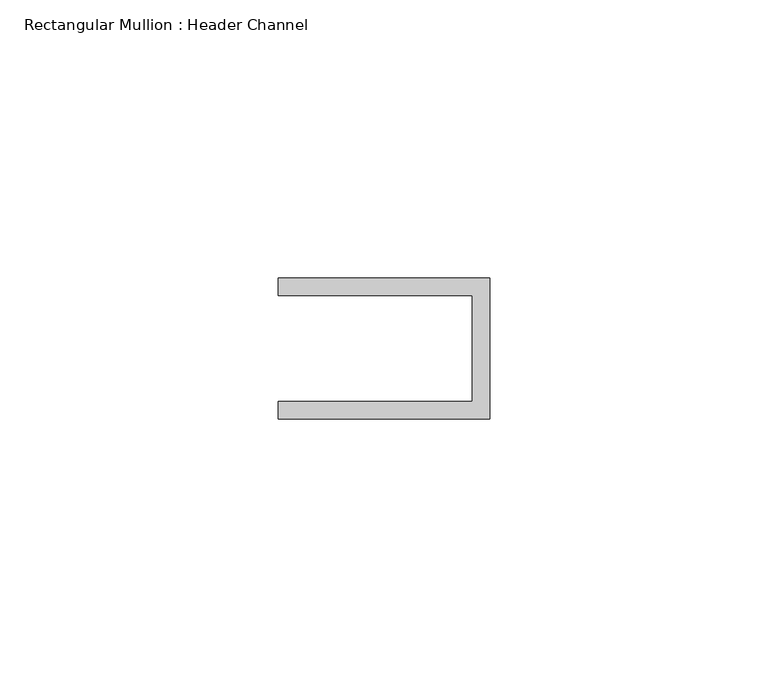
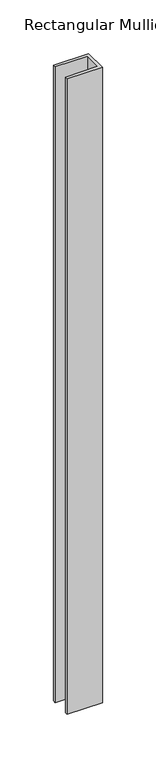
"""IFC4 building model written with IfcOpenShell, lengths in millimetres: member geometry, Rectangular Mullion : Header Channel."""

from ifc_helpers import new_model, si_unit, frame, origin, place, context, project, spatial, polyline, outline, extrude, source, transform, mapped, element, save


def rectangular_mullion_header_channel_e476e37a(model_context):
    return source(origin(), model_context, "Body", "SweptSolid", [
        extrude(outline(polyline([(0.0, -12.7), (-38.1, -12.7), (-38.1, -9.525), (-3.175, -9.525), (-3.175, 9.525), (-38.1, 9.525), (-38.1, 12.7), (0.0, 12.7), (0.0, -12.7)])), frame((0.0, 0.0, -723.9), z_axis=(0.0, 0.0, 1.0), x_axis=(1.0, 0.0, 0.0)), (0.0, 0.0, 1.0), 723.9),
    ])


if __name__ == "__main__":
    model = new_model("IFC4")
    model_context = context("Model", 3, world=origin())
    ifc_project = project(units=[si_unit("LENGTHUNIT", "METRE", prefix="MILLI")], contexts=[model_context])
    site = spatial("IfcSite", under=ifc_project)
    building = spatial("IfcBuilding", under=site)
    placement = place(None, origin())
    rectangular_mullion_header_channel_shape = rectangular_mullion_header_channel_e476e37a(model_context)
    element("IfcMember", 1, ObjectType="Rectangular Mullion : Header Channel", at=placement, inside=building, context=model_context, shape_type="MappedRepresentation", body=[
        mapped(rectangular_mullion_header_channel_shape, transform((0.0, 0.0, 0.0), x_axis=(1.0, 0.0, 0.0), y_axis=(0.0, 1.0, 0.0), z_axis=(0.0, 0.0, 1.0))),
    ])
    save(model, "model.ifc")

# Revit data of these elements
# Type "Rectangular Mullion : Header Channel"
#   built-in parameter 1007322 = 0.0833333 (stored number, unit not read)
#   built-in parameter 1007321 = -0.03125 (stored number, unit not read)
#   built-in parameter 1007320 = 0.0416667 (stored number, unit not read)
# Element 1 (IfcMember, "Rectangular Mullion : Header Channel")
#   Materials on its faces: "ALUM"
# Materials
#   "ALUM": class "Generic", colour RGB 157 157 157, transparency 0, Cost = 0
